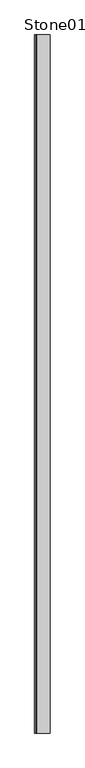
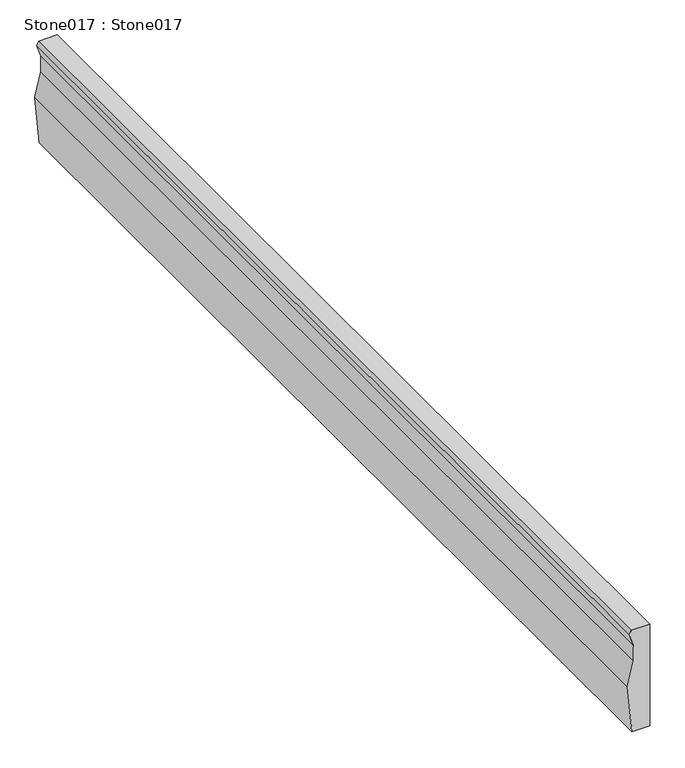
"""IFC4 building model written with IfcOpenShell, lengths in millimetres: proxy geometry, Stone017 : Stone017."""

import ifcopenshell
import ifcopenshell.guid

model = None  # the IFC model being written
_history = None  # IfcOwnerHistory: only IFC2X3 demands one
_inside = {}  # id of a spatial element -> (the spatial element, [elements in it])
_under = {}  # id of a project, library or spatial element -> (it, [spatial elements below it])
_declared = {}  # id of a project -> (the project, [libraries it declares])
_typed = {}  # id of a type object -> (the type object, [elements of that type])
_made_of = {}  # id of a material, layer set ... -> (it, [elements and type objects made of it])


def new_model(schema):
    """Start an empty IFC model of exactly this schema.

    Asked for "IFC4X3", IfcOpenShell would pick the latest addendum, in which some entities
    have other attributes; the version numbers below select the first issue.
    IFC2X3 requires an IfcOwnerHistory on every rooted entity: one is made here for all.
    """
    global model, _history
    if schema == "IFC4X3":
        model = ifcopenshell.file(schema_version=(4, 3, 0, 0))
    else:
        model = ifcopenshell.file(schema=schema)
    _inside.clear()
    _under.clear()
    _declared.clear()
    _typed.clear()
    _made_of.clear()
    _history = None
    if model.schema == "IFC2X3":
        org = make("IfcOrganization", Name="unknown")
        user = make(
            "IfcPersonAndOrganization",
            ThePerson=make("IfcPerson", FamilyName="unknown"),
            TheOrganization=org,
        )
        app = make(
            "IfcApplication",
            ApplicationDeveloper=org,
            Version="unknown",
            ApplicationFullName="unknown",
            ApplicationIdentifier="unknown",
        )
        _history = make(
            "IfcOwnerHistory",
            OwningUser=user,
            OwningApplication=app,
            ChangeAction="ADDED",
            CreationDate=0,
        )
    return model


def make(cls, **values):
    """One entity of the class cls with the attributes given. An attribute that is None is left unset."""
    return model.create_entity(
        cls, **{name: value for name, value in values.items() if value is not None}
    )


def rooted(cls, **values):
    """An entity with a GlobalId (a new one), such as an element, a storey or a relation."""
    return make(cls, GlobalId=ifcopenshell.guid.new(), OwnerHistory=_history, **values)


def si_unit(unit_type, name, prefix=None):
    """IfcSIUnit, for example si_unit("LENGTHUNIT", "METRE", prefix="MILLI")."""
    return make("IfcSIUnit", UnitType=unit_type, Prefix=prefix, Name=name)


def assignment(units):
    """IfcUnitAssignment: the units of a project."""
    return None if units is None else make("IfcUnitAssignment", Units=units)


def point(xyz):
    """IfcCartesianPoint."""
    return None if xyz is None else make("IfcCartesianPoint", Coordinates=xyz)


def direction(xyz):
    """IfcDirection."""
    return None if xyz is None else make("IfcDirection", DirectionRatios=xyz)


def frame(location, z_axis=None, x_axis=None):
    """IfcAxis2Placement3D, a coordinate frame: its origin and axes. An axis left out is left unset."""
    return make(
        "IfcAxis2Placement3D",
        Location=point(location),
        Axis=direction(z_axis),
        RefDirection=direction(x_axis),
    )


def origin():
    """The frame at (0, 0, 0) with its axes left unset."""
    return frame((0.0, 0.0, 0.0))


def place(relative_to, where):
    """IfcLocalPlacement: puts the frame where relative to a parent placement (None: the world)."""
    return make(
        "IfcLocalPlacement", PlacementRelTo=relative_to, RelativePlacement=where
    )


def context(
    kind, dimensions, precision=None, world=None, true_north=None, identifier=None
):
    """IfcGeometricRepresentationContext, for example the 3D "Model" context."""
    return make(
        "IfcGeometricRepresentationContext",
        ContextIdentifier=identifier,
        ContextType=kind,
        CoordinateSpaceDimension=dimensions,
        Precision=precision,
        WorldCoordinateSystem=world,
        TrueNorth=true_north,
    )


def project(units=None, contexts=None):
    """IfcProject with its units and contexts."""
    return rooted(
        "IfcProject",
        Name="project",
        RepresentationContexts=contexts,
        UnitsInContext=assignment(units),
    )


def spatial(cls, under=None, at=None, **own):
    """A site, building, storey or space (cls), placed at a placement, below another one or the project."""
    s = rooted(cls, ObjectPlacement=at, **own)
    if under is not None:
        _under.setdefault(under.id(), (under, []))[1].append(s)
    return s


def polyline(points):
    """IfcPolyline through the points."""
    return make("IfcPolyline", Points=[point(p) for p in points])


def outline(outer, holes=None, kind="AREA"):
    """IfcArbitraryClosedProfileDef: a profile drawn as a closed curve; with holes, ...WithVoids."""
    if holes is None:
        return make("IfcArbitraryClosedProfileDef", ProfileType=kind, OuterCurve=outer)
    return make(
        "IfcArbitraryProfileDefWithVoids",
        ProfileType=kind,
        OuterCurve=outer,
        InnerCurves=holes,
    )


def extrude(swept, where, along, depth):
    """IfcExtrudedAreaSolid: the profile swept, set in the frame where, extruded along a direction by depth."""
    return make(
        "IfcExtrudedAreaSolid",
        SweptArea=swept,
        Position=where,
        ExtrudedDirection=direction(along),
        Depth=depth,
    )


def shape(context_of_items, identifier, shape_type, items):
    """IfcShapeRepresentation: the items that make up one representation, for example the "Body"."""
    return make(
        "IfcShapeRepresentation",
        ContextOfItems=context_of_items,
        RepresentationIdentifier=identifier,
        RepresentationType=shape_type,
        Items=items,
    )


def source(mapping_origin, context_of_items, identifier, shape_type, items):
    """IfcRepresentationMap: a shape defined once, which mapped items show again and again."""
    return make(
        "IfcRepresentationMap",
        MappingOrigin=mapping_origin,
        MappedRepresentation=shape(context_of_items, identifier, shape_type, items),
    )


def transform(
    local_origin,
    x_axis=None,
    y_axis=None,
    z_axis=None,
    scale=None,
    scale2=None,
    scale3=None,
    uniform=True,
):
    """IfcCartesianTransformationOperator3D, or its non-uniform kind. x_axis, y_axis, z_axis: its Axis1, 2, 3."""
    if uniform:
        return make(
            "IfcCartesianTransformationOperator3D",
            Axis1=direction(x_axis),
            Axis2=direction(y_axis),
            LocalOrigin=point(local_origin),
            Scale=scale,
            Axis3=direction(z_axis),
        )
    return make(
        "IfcCartesianTransformationOperator3DnonUniform",
        Axis1=direction(x_axis),
        Axis2=direction(y_axis),
        LocalOrigin=point(local_origin),
        Scale=scale,
        Axis3=direction(z_axis),
        Scale2=scale2,
        Scale3=scale3,
    )


def mapped(mapping_source, mapping_target):
    """IfcMappedItem: shows the shape of a source again, moved by a transform."""
    return make(
        "IfcMappedItem", MappingSource=mapping_source, MappingTarget=mapping_target
    )


def made_of(thing, what):
    """Note that an element or type object is made of a material, layer set ...; save() writes the relation."""
    if what is not None:
        _made_of.setdefault(what.id(), (what, []))[1].append(thing)
    return thing


def element(
    cls,
    number,
    at=None,
    inside=None,
    cuts=None,
    type_object=None,
    material=None,
    context=None,
    identifier="Body",
    shape_type=None,
    held_by="IfcProductDefinitionShape",
    body=None,
    shapes=None,
    **own,
):
    """One element of the class cls, such as IfcWall. Its Tag is "e" and its number.

    at: its placement. inside: the storey or other place that contains it. cuts: it is an
    opening in that element (IfcRelVoidsElement). A single representation is given by context,
    identifier, shape_type and body (its items); several are given by shapes. held_by: the class
    of the entity that holds the representations. save() writes the other relations.
    """
    e = rooted(cls, Tag="e%d" % number, ObjectPlacement=at, **own)
    if body is not None:
        shapes = [shape(context, identifier, shape_type, body)]
    if shapes is not None:
        e.Representation = make(held_by, Representations=shapes)
    if inside is not None:
        _inside.setdefault(inside.id(), (inside, []))[1].append(e)
    if cuts is not None:
        rooted(
            "IfcRelVoidsElement", RelatingBuildingElement=cuts, RelatedOpeningElement=e
        )
    if type_object is not None:
        _typed.setdefault(type_object.id(), (type_object, []))[1].append(e)
    return made_of(e, material)


def aggregate(whole, parts):
    """IfcRelAggregates: a whole, such as a stair, and the parts it consists of."""
    return rooted("IfcRelAggregates", RelatingObject=whole, RelatedObjects=parts)


def save(model, path):
    """Write the relations noted so far, then the file.

    IfcRelAggregates (storeys below a building ...), IfcRelContainedInSpatialStructure (elements
    in a storey), IfcRelDefinesByType, IfcRelAssociatesMaterial and IfcRelDeclares: one each for
    every whole, place, type object, material and project.
    """
    for whole, parts in _under.values():
        aggregate(whole, parts)
    for where, things in _inside.values():
        rooted(
            "IfcRelContainedInSpatialStructure",
            RelatedElements=things,
            RelatingStructure=where,
        )
    for kind, things in _typed.values():
        rooted("IfcRelDefinesByType", RelatedObjects=things, RelatingType=kind)
    for what, things in _made_of.values():
        rooted("IfcRelAssociatesMaterial", RelatedObjects=things, RelatingMaterial=what)
    for by, libraries in _declared.values():
        rooted("IfcRelDeclares", RelatingContext=by, RelatedDefinitions=libraries)
    model.write(path)


def stone017_stone017_f5c83055(model_context):
    return source(origin(), model_context, "Body", "SweptSolid", [
        extrude(outline(polyline([(33394.2430685, -10302.7509766), (33385.90625, -10305.9892578), (33362.4765625, -10298.8007813), (33330.0664062, -10298.3115234), (33280.7148437, -10309.8115234), (33185.140625, -10301.6737014), (33185.140625, -10266.1494141), (33394.2430685, -10266.1494141), (33394.2430685, -10302.7509766)])), frame((0.0, 7982.1531721, 0.0), z_axis=(0.0, 1.0, 0.0), x_axis=(0.0, 0.0, 1.0)), (0.0, 0.0, 1.0), 2000.0),
    ])


if __name__ == "__main__":
    model = new_model("IFC4")
    model_context = context("Model", 3, world=origin())
    ifc_project = project(units=[si_unit("LENGTHUNIT", "METRE", prefix="MILLI")], contexts=[model_context])
    site = spatial("IfcSite", under=ifc_project)
    building = spatial("IfcBuilding", under=site)
    placement = place(None, origin())
    stone017_stone017_shape = stone017_stone017_f5c83055(model_context)
    element("IfcBuildingElementProxy", 1, Name="Stone017 : Stone017", ObjectType="Stone017 : Stone017", at=placement, inside=building, context=model_context, shape_type="MappedRepresentation", body=[
        mapped(stone017_stone017_shape, transform((0.0, 0.0, 0.0), x_axis=(1.0, 0.0, 0.0), y_axis=(0.0, 1.0, 0.0), z_axis=(0.0, 0.0, 1.0))),
    ])
    save(model, "model.ifc")

# Revit data of these elements
# Type "Stone017 : Stone017"
#   NameOverride = "Stone017"
# Element 1 (IfcBuildingElementProxy, "Stone017 : Stone017")
#   Materials on its faces: "SPLIT FACE STONE 1032"
# Materials
#   "SPLIT FACE STONE 1032": class "Unassigned", colour RGB 205 195 181, transparency 0
